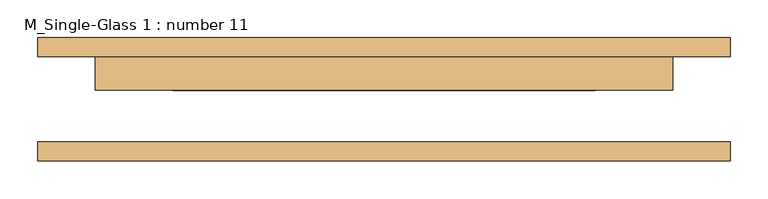
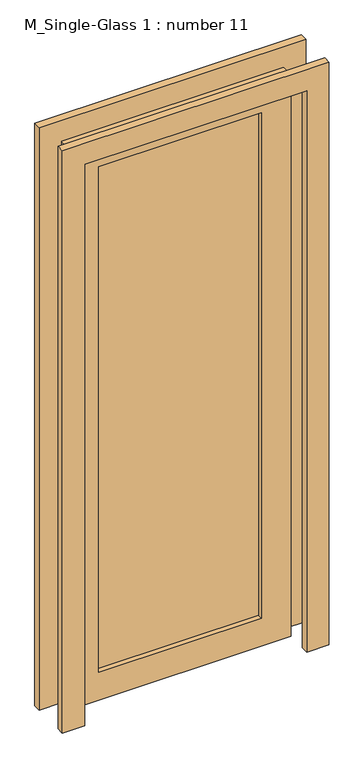
"""IFC4 building model written with IfcOpenShell, lengths in millimetres: door geometry, M_Single-Glass 1 : number 11."""

from ifc_helpers import new_model, si_unit, frame, origin, place, context, project, spatial, polyline, outline, extrude, source, transform, mapped, element, save


def m_single_glass_1_number_11_6cc171e0(model_context):
    return source(origin(), model_context, "Body", "SweptSolid", [
        extrude(outline(polyline([(2032.0, 381.0), (0.0, 381.0), (0.0, 457.0), (2108.0, 457.0), (2108.0, -457.0), (0.0, -457.0), (0.0, -381.0), (2032.0, -381.0), (2032.0, 381.0)])), frame((0.0, -81.35625, 0.0), z_axis=(0.0, 1.0, 0.0), x_axis=(0.0, 0.0, 1.0)), (0.0, 0.0, 1.0), 25.0),
        extrude(outline(polyline([(2032.0, 381.0), (0.0, 381.0), (0.0, 457.0), (2108.0, 457.0), (2108.0, -457.0), (0.0, -457.0), (0.0, -381.0), (2032.0, -381.0), (2032.0, 381.0)])), frame((0.0, 56.35625, 0.0), z_axis=(0.0, 1.0, 0.0), x_axis=(0.0, 0.0, 1.0)), (0.0, 0.0, 1.0), 25.0),
        extrude(outline(polyline([(279.0, 27.78125), (-279.0, 27.78125), (-279.0, 34.13125), (279.0, 34.13125), (279.0, 27.78125)])), frame((0.0, 0.0, 102.0), z_axis=(0.0, 0.0, 1.0), x_axis=(1.0, 0.0, 0.0)), (0.0, 0.0, 1.0), 1828.0),
        extrude(outline(polyline([(2032.0, 381.0), (2032.0, -381.0), (0.0, -381.0), (0.0, 381.0), (2032.0, 381.0)]), holes=[polyline([(1930.0, -279.0), (1930.0, 279.0), (102.0, 279.0), (102.0, -279.0), (1930.0, -279.0)])]), frame((0.0, 11.90625, 0.0), z_axis=(0.0, 1.0, 0.0), x_axis=(0.0, 0.0, 1.0)), (0.0, 0.0, 1.0), 44.45),
    ])


if __name__ == "__main__":
    model = new_model("IFC4")
    model_context = context("Model", 3, world=origin())
    ifc_project = project(units=[si_unit("LENGTHUNIT", "METRE", prefix="MILLI")], contexts=[model_context])
    site = spatial("IfcSite", under=ifc_project)
    building = spatial("IfcBuilding", under=site)
    placement = place(None, origin())
    m_single_glass_1_number_11_shape = m_single_glass_1_number_11_6cc171e0(model_context)
    element("IfcDoor", 1, ObjectType="M_Single-Glass 1 : number 11", at=placement, inside=building, context=model_context, shape_type="MappedRepresentation", body=[
        mapped(m_single_glass_1_number_11_shape, transform((0.0, 0.0, 0.0), x_axis=(1.0, 0.0, 0.0), y_axis=(0.0, 1.0, 0.0), z_axis=(0.0, 0.0, 1.0))),
    ])
    save(model, "model.ifc")

# Revit data of these elements
# Type "M_Single-Glass 1 : number 11"
#   Type Mark = "123"
#   Thickness = 0' - 1 3/4"
#   Height = 6' - 8"
#   Rail Width - Base = 0' - 4.01575"
#   Rail Width - Top = 0' - 4.01575"
#   Stile Width - Hinge = 0' - 4.01575"
#   Stile Width - Latch = 0' - 4.01575"
#   Trim Projection Ext = 0' - 0.98425"
#   Trim Projection Int = 0' - 0.98425"
#   Trim Width = 0' - 2.99213"
#   Width = 2' - 6"
#   Door Material = Door - Panel
#   Frame Material = Door - Frame
#   Function = (empty or 0)
#   Wall Closure = (empty or 0)
# Element 1 (IfcDoor, "M_Single-Glass 1 : number 11")
#   Materials on its faces: "Door - Frame", "Door - Panel", "Glass"
# Materials
#   "Door - Panel": class "Wood", colour RGB 210 159 95, transparency 0, Keynote = "L20", Cost = 0
#   "Door - Frame": class "Miscellaneous", colour RGB 118 70 51, transparency 0
#   "Glass": class "Glass", colour RGB 0 128 192, transparency 0.9, Description = "Soda Lime Glass", Cost = 0
